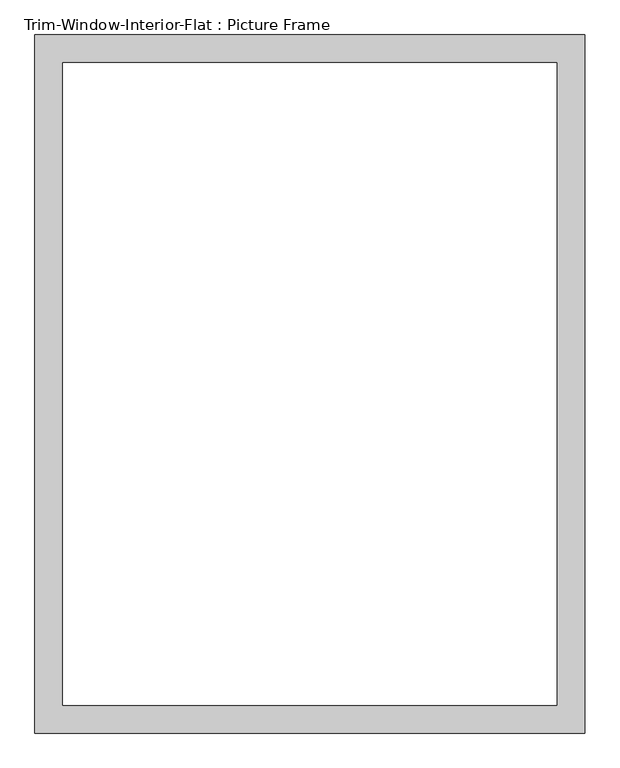
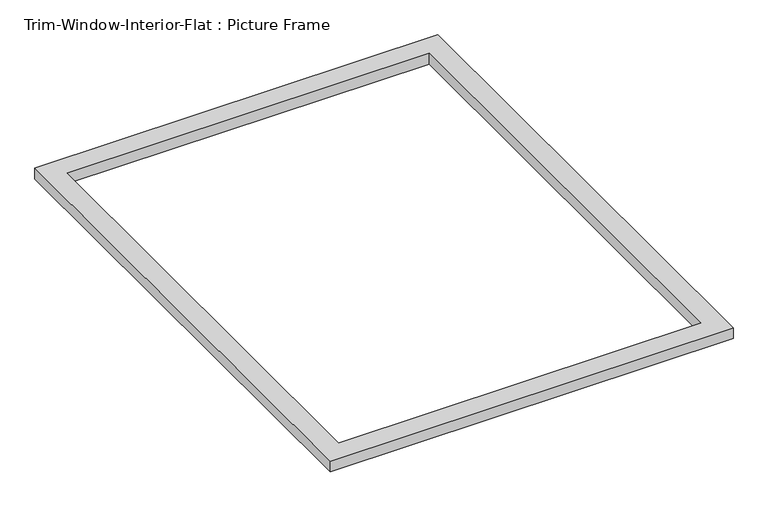
"""IFC4 building model written with IfcOpenShell, lengths in millimetres: proxy geometry, Trim-Window-Interior-Flat : Picture Frame."""

from ifc_helpers import new_model, si_unit, origin, origin_with_axes, place, context, project, spatial, polyline, outline, extrude, source, transform, mapped, element, save


def trim_window_interior_flat_picture_frame_cf41f3d5(model_context):
    return source(origin(), model_context, "Body", "SweptSolid", [
        extrude(outline(polyline([(565.15, -44.45), (-565.15, -44.45), (-565.15, 1390.65), (565.15, 1390.65), (565.15, -44.45)]), holes=[polyline([(508.0, 12.7), (508.0, 1333.5), (-508.0, 1333.5), (-508.0, 12.7), (508.0, 12.7)])]), origin_with_axes(), (0.0, 0.0, 1.0), 31.75),
    ])


if __name__ == "__main__":
    model = new_model("IFC4")
    model_context = context("Model", 3, world=origin())
    ifc_project = project(units=[si_unit("LENGTHUNIT", "METRE", prefix="MILLI")], contexts=[model_context])
    site = spatial("IfcSite", under=ifc_project)
    building = spatial("IfcBuilding", under=site)
    placement = place(None, origin())
    trim_window_interior_flat_picture_frame_shape = trim_window_interior_flat_picture_frame_cf41f3d5(model_context)
    element("IfcBuildingElementProxy", 1, Name="Trim-Window-Interior-Flat : Picture Frame", ObjectType="Trim-Window-Interior-Flat : Picture Frame", at=placement, inside=building, context=model_context, shape_type="MappedRepresentation", body=[
        mapped(trim_window_interior_flat_picture_frame_shape, transform((0.0, 0.0, 0.0), x_axis=(1.0, 0.0, 0.0), y_axis=(0.0, 1.0, 0.0), z_axis=(0.0, 0.0, 1.0))),
    ])
    save(model, "model.ifc")

# Revit data of these elements
# Type "Trim-Window-Interior-Flat : Picture Frame"
#   Trim Thickness_Picture Frame = 0' - 1 1/4"
#   Trim Width = 0' - 2 1/4"
#   Trim Thickness_with Sill = 0' - 0 3/4"
#   Sill Thickness = 0' - 1 1/4"
#   Opening Width [instance default] = 2' - 0"
#   Opening Height [instance default] = 3' - 0"
#   Default Elevation = 4' - 0"
#   Sill = no
#   Picture Frame = yes
#   Trim Material [instance default] = none
# Element 1 (IfcBuildingElementProxy, "Trim-Window-Interior-Flat : Picture Frame")
#   Opening Width = 3' - 5"
#   Opening Height = 4' - 5"
#   Trim Material = Wood - Stained
#   Materials on its faces: "Wood - Stained"
# Materials
#   "Wood - Stained": class "Wood", colour RGB 224 178 126, transparency 0, Cost = 0
